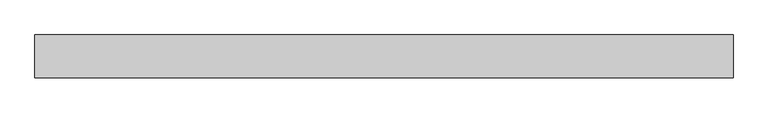
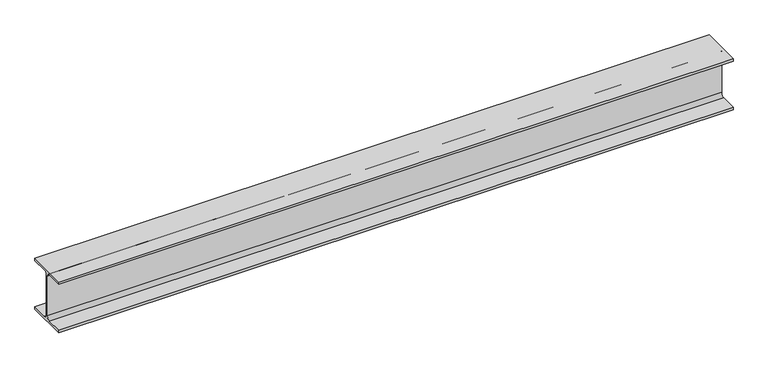
"""IFC4 building model written with IfcOpenShell, lengths in millimetres: beam geometry, 0912_Steel Framing_H-KSD3502 : H_SB_ASB_H-194x150x6x9."""

from ifc_helpers import new_model, si_unit, point, frame, frame_2d, origin, place, context, project, spatial, polyline, circle_curve, trimmed, segment, composite_curve, outline, extrude, source, transform, mapped, element, save


def beam_4ffcef56(model_context):
    return source(origin(), model_context, "Body", "SweptSolid", [
        extrude(outline(composite_curve([segment(polyline([(-75.0, -88.0), (-16.0, -88.0)]), True, "CONTINUOUS"), segment(trimmed(circle_curve(frame_2d((-16.0, -75.0)), 13.0), [point((-16.0, -88.0))], [point((-3.0, -75.0))], True, "CARTESIAN"), True, "CONTINUOUS"), segment(polyline([(-3.0, -75.0), (-3.0, 75.0)]), True, "CONTINUOUS"), segment(trimmed(circle_curve(frame_2d((-16.0, 75.0)), 13.0), [point((-3.0, 75.0))], [point((-16.0, 88.0))], True, "CARTESIAN"), True, "CONTINUOUS"), segment(polyline([(-16.0, 88.0), (-75.0, 88.0), (-75.0, 97.0), (75.0, 97.0), (75.0, 88.0), (16.0, 88.0)]), True, "CONTINUOUS"), segment(trimmed(circle_curve(frame_2d((16.0, 75.0)), 13.0), [point((16.0, 88.0))], [point((3.0, 75.0))], True, "CARTESIAN"), True, "CONTINUOUS"), segment(polyline([(3.0, 75.0), (3.0, -75.0)]), True, "CONTINUOUS"), segment(trimmed(circle_curve(frame_2d((16.0, -75.0)), 13.0), [point((3.0, -75.0))], [point((16.0, -88.0))], True, "CARTESIAN"), True, "CONTINUOUS"), segment(polyline([(16.0, -88.0), (75.0, -88.0), (75.0, -97.0), (-75.0, -97.0), (-75.0, -88.0)]), True, "CONTINUOUS")], self_intersect=False)), frame((-1200.0, 0.0, 0.0), z_axis=(1.0, 0.0, 0.0), x_axis=(0.0, 1.0, 0.0)), (0.0, 0.0, 1.0), 2433.3704936),
    ])


if __name__ == "__main__":
    model = new_model("IFC4")
    model_context = context("Model", 3, world=origin())
    ifc_project = project(units=[si_unit("LENGTHUNIT", "METRE", prefix="MILLI")], contexts=[model_context])
    site = spatial("IfcSite", under=ifc_project)
    building = spatial("IfcBuilding", under=site)
    placement = place(None, origin())
    beam_shape = beam_4ffcef56(model_context)
    element("IfcBeam", 1, ObjectType="0912_Steel Framing_H-KSD3502 : H_SB_ASB_H-194x150x6x9", at=placement, inside=building, context=model_context, shape_type="MappedRepresentation", body=[
        mapped(beam_shape, transform((0.0, 0.0, 0.0), x_axis=(1.0, 0.0, 0.0), y_axis=(0.0, 1.0, 0.0), z_axis=(0.0, 0.0, 1.0))),
    ])
    save(model, "model.ifc")

# Revit data of these elements
# Type "0912_Steel Framing_H-KSD3502 : H_SB_ASB_H-194x150x6x9"
#   H_WM Code_1 = "S01AA002-00001 | Main Steel Structure Fabrication Work | Shelter/Building | Medium Steel - Standard (90KG/M>Weight≥30KG/M) | Material: (   )"
#   H_WM Code_2 = "S03AA028-00001 | Main Steel Structure Erection Work | Shelter/Building | Medium Steel (90KG/M>Weight≥30KG/M) | Material: (   )"
#   H_WM Code_3 = "S01AA010-00001 | Main Steel Structure Fabrication Work | Shelter/Building | Steel Painting/Coating | for Non-Fireproofed Steel Surface, Surface Preparation, Primer, Second & Final Coat | Material: (   )"
#   H_Q'ty Cal Type Tag = "SB-Q2"
#   Width = 15.0 cm
#   Web Thickness = 0.6 cm
#   Web Fillet = 1.3 cm
#   Warping Constant = 43316.0 cm⁶
#   W = 0
#   Torsional Moment of Inertia = 8.622 cm⁴
#   Section Area = 39.01 cm²
#   Plastic Modulus weak axis = 104.0 cm³
#   Plastic Modulus strong axis = 309.0 cm³
#   Perimeter = 0.95 m²/m
#   Nominal Weight = 30.60 kgf/m
#   Moment of Inertia weak axis = 507.00 cm⁴
#   Moment of Inertia strong axis = 2690.00 cm⁴
#   Height = 19.4 cm
#   Flange Thickness = 0.9 cm
#   Elastic Modulus weak axis = 67.6 cm³
#   Elastic Modulus strong axis = 277.0 cm³
#   Centroid Vertical = 9.7 cm
#   Centroid Horizontal = 7.5 cm
#   Ix = 26900000
#   Length [instance default] = 1.5240 m
#   Zx = 309000
#   b = 0.1500 m
#   h = 0.1940 m
#   r = 0.0130 m
#   s = 0.0060 m
#   t = 0.0090 m
#   A = 0.003901 m²
#   Structural Material [instance default] = Steel, 45-345
#   Assembly Code = ""
# Element 1 (IfcBeam, "0912_Steel Framing_H-KSD3502 : H_SB_ASB_H-194x150x6x9")
#   Structural Material = none
# Materials
#   "Steel, 45-345": class "Metal", colour RGB 189 187 185, transparency 0, Description = "Steel 345 MPa", Cost = 0
